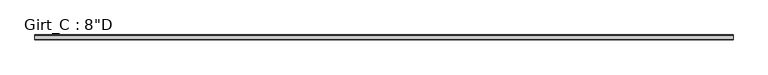
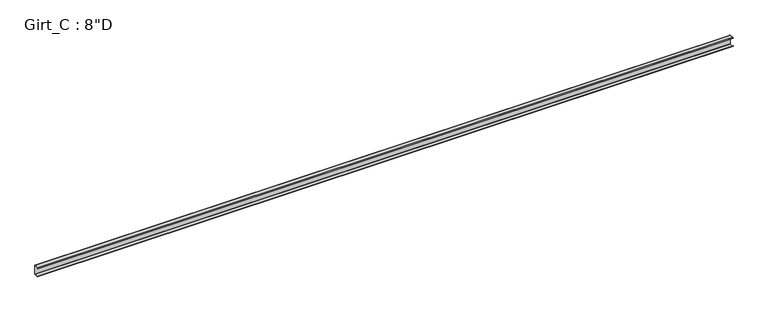
"""IFC4 building model written with IfcOpenShell, lengths in millimetres: beam geometry."""

from ifc_helpers import new_model, si_unit, point, frame, frame_2d, origin, place, context, project, spatial, polyline, circle_curve, trimmed, segment, composite_curve, outline, extrude, source, transform, mapped, element, save


def beam_fff442ec(model_context):
    return source(origin(), model_context, "Body", "SweptSolid", [
        extrude(outline(composite_curve([segment(polyline([(-87.5109375, 101.6), (-3.3734375, 101.6)]), True, "CONTINUOUS"), segment(trimmed(circle_curve(frame_2d((-3.3734375, 96.8375)), 4.7625), [point((-3.3734375, 101.6))], [point((1.3890625, 96.8375))], False, "CARTESIAN"), True, "CONTINUOUS"), segment(polyline([(1.3890625, 96.8375), (1.3890625, -96.8375)]), True, "CONTINUOUS"), segment(trimmed(circle_curve(frame_2d((-3.3734375, -96.8375)), 4.7625), [point((1.3890625, -96.8375))], [point((-3.3734375, -101.6))], False, "CARTESIAN"), True, "CONTINUOUS"), segment(polyline([(-3.3734375, -101.6), (-87.5109375, -101.6), (-99.7792647, -86.979177), (-97.6510975, -85.1934327), (-86.2154765, -98.821875), (-3.2694106, -98.821875)]), True, "CONTINUOUS"), segment(trimmed(circle_curve(frame_2d((-3.3748024, -96.8389339)), 1.9857399), [point((-3.2694106, -98.821875))], [point((-1.3890625, -96.8389339))], True, "CARTESIAN"), True, "CONTINUOUS"), segment(polyline([(-1.3890625, -96.8389339), (-1.3890625, 96.8381931)]), True, "CONTINUOUS"), segment(trimmed(circle_curve(frame_2d((-3.3741066, 96.8381931)), 1.9850441), [point((-1.3890625, 96.8381931))], [point((-3.3005807, 98.821875))], True, "CARTESIAN"), True, "CONTINUOUS"), segment(polyline([(-3.3005807, 98.821875), (-86.2154765, 98.821875), (-97.6278742, 85.221109), (-99.7560415, 87.0068534), (-87.5109375, 101.6)]), True, "CONTINUOUS")], self_intersect=False)), frame((-7342.584375, 0.0, 0.0), z_axis=(1.0, 0.0, 0.0), x_axis=(0.0, 1.0, 0.0)), (0.0, 0.0, 1.0), 14674.85),
    ])


if __name__ == "__main__":
    model = new_model("IFC4")
    model_context = context("Model", 3, world=origin())
    ifc_project = project(units=[si_unit("LENGTHUNIT", "METRE", prefix="MILLI")], contexts=[model_context])
    site = spatial("IfcSite", under=ifc_project)
    building = spatial("IfcBuilding", under=site)
    placement = place(None, origin())
    beam_shape = beam_fff442ec(model_context)
    element("IfcBeam", 1, ObjectType="Girt_C : 8\"D", at=placement, inside=building, context=model_context, shape_type="MappedRepresentation", body=[
        mapped(beam_shape, transform((0.0, 0.0, 0.0), x_axis=(1.0, 0.0, 0.0), y_axis=(0.0, 1.0, 0.0), z_axis=(0.0, 0.0, 1.0))),
    ])
    save(model, "model.ifc")

# Revit data of these elements
# Type "Girt_C : 8\"D"
#   half leg = 0' - 1 3/4"
#   Web_Thickness = 0' - 0 7/64"
#   Length [instance default] = 10' - 0"
#   Leg_1 = 0' - 3 1/2"
#   Height = 0' - 8"
#   Structural Material [instance default] = none
# Element 1 (IfcBeam, "Girt_C : 8\"D")
#   Structural Material = GALVANIZED 'CEE' SECTION (8.0x3.5C - SEE STRUCT. DWGS)
#   Materials on its faces: "GALVANIZED 'CEE' SECTION (8.0x3.5C - SEE STRUCT. DWGS)"
# Materials
#   "GALVANIZED 'CEE' SECTION (8.0x3.5C - SEE STRUCT. DWGS)": class "Metal", colour RGB 137 146 153, transparency 0, Description = "Steel, mill finish", Cost = 0
